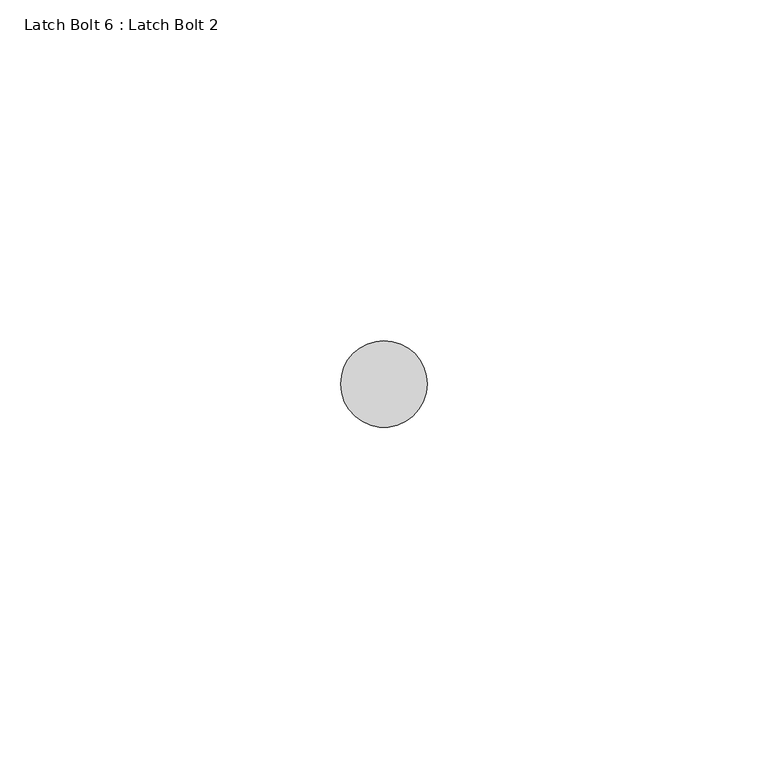
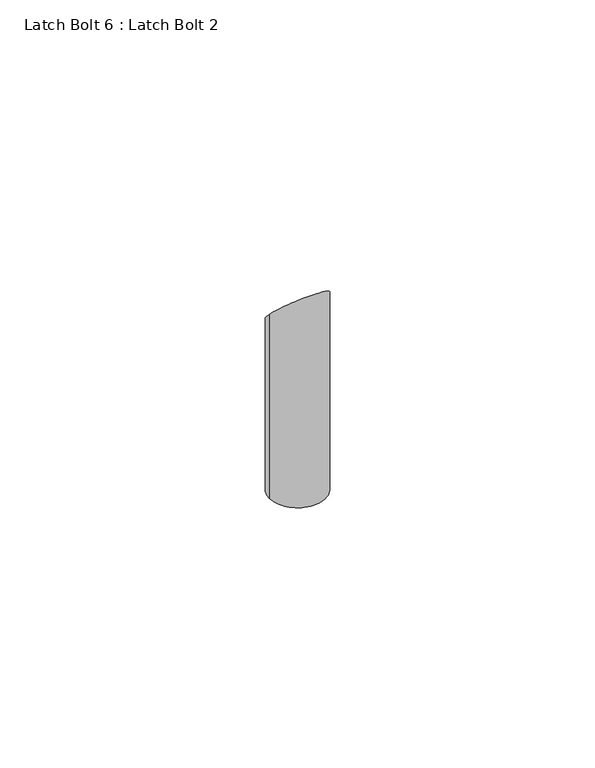
"""IFC4 building model written with IfcOpenShell, lengths in millimetres: proxy geometry, Latch Bolt 6 : Latch Bolt 2."""

from ifc_helpers import new_model, si_unit, frame, origin, place, context, project, spatial, circle_curve, ellipse_curve, source, transform, mapped, element, save
from ifc_brep_helpers import plane_surface, cylinder_surface, advanced_brep


def latch_bolt_6_latch_bolt_2_5f3dc6ce(model_context):
    return source(origin(), model_context, "Body", "AdvancedBrep", [
        advanced_brep(
        [(587306.3384816, -535293.641467, 1022.35), (587319.0384816, -535293.641467, 1022.35), (587319.0384816, -535293.641467, 1066.7505507), (587306.3384816, -535293.641467, 1066.7505507), (587312.6884816, -535287.291467, 1060.4005507)],
        [
            (0, 1, circle_curve(frame((587312.6884816, -535293.641467, 1022.35), z_axis=(0.0, 0.0, -1.0), x_axis=(1.0, 0.0, 0.0)), 6.35)),
            (1, 0, circle_curve(frame((587312.6884816, -535293.641467, 1022.35), z_axis=(0.0, 0.0, -1.0), x_axis=(1.0, 0.0, 0.0)), 6.35)),
            (1, 2),
            (2, 3, ellipse_curve(frame((587312.6884816, -535293.641467, 1066.7505507), z_axis=(0.0, -0.7071067811861375, -0.7071067811869577), x_axis=(0.0, -0.7071067811869577, 0.7071067811861372)), 8.9802561, 6.35)),
            (3, 0),
            (3, 4, ellipse_curve(frame((587312.6884816, -535293.641467, 1066.7505507), z_axis=(0.0, -0.7071067811861375, -0.7071067811869577), x_axis=(0.0, -0.7071067811869577, 0.7071067811861372)), 8.9802561, 6.35)),
            (4, 2, ellipse_curve(frame((587312.6884816, -535293.641467, 1066.7505507), z_axis=(0.0, -0.7071067811861375, -0.7071067811869577), x_axis=(0.0, -0.7071067811869577, 0.7071067811861372)), 8.9802561, 6.35)),
        ],
        [
            plane_surface(frame((587319.0384816, -535293.641467, 1022.35), z_axis=(0.0, 0.0, -1.0), x_axis=(0.0, -1.0, 0.0))),
            cylinder_surface(frame((587312.6884816, -535293.641467, 1022.35), z_axis=(0.0, 0.0, 1.0), x_axis=(1.0, 0.0, 0.0)), 6.35),
            plane_surface(frame((587338.1185739, -535303.166467, 1076.2755507), z_axis=(0.0, 0.7071067811861375, 0.7071067811869577), x_axis=(-1.0, 0.0, 0.0))),
        ],
        [
            (0, [[1, 2]]),
            (1, [[-2, 3, 4, 5]]),
            (1, [[-1, -5, 6, 7, -3]]),
            (2, [[-4, -7, -6]]),
        ],
    ),
    ])


if __name__ == "__main__":
    model = new_model("IFC4")
    model_context = context("Model", 3, world=origin())
    ifc_project = project(units=[si_unit("LENGTHUNIT", "METRE", prefix="MILLI")], contexts=[model_context])
    site = spatial("IfcSite", under=ifc_project)
    building = spatial("IfcBuilding", under=site)
    placement = place(None, origin())
    latch_bolt_6_latch_bolt_2_shape = latch_bolt_6_latch_bolt_2_5f3dc6ce(model_context)
    element("IfcBuildingElementProxy", 1, Name="Latch Bolt 6 : Latch Bolt 2", ObjectType="Latch Bolt 6 : Latch Bolt 2", at=placement, inside=building, context=model_context, shape_type="MappedRepresentation", body=[
        mapped(latch_bolt_6_latch_bolt_2_shape, transform((0.0, 0.0, 0.0), x_axis=(1.0, 0.0, 0.0), y_axis=(0.0, 1.0, 0.0), z_axis=(0.0, 0.0, 1.0))),
    ])
    save(model, "model.ifc")

# Revit data of these elements
# Element 1 (IfcBuildingElementProxy, "Latch Bolt 6 : Latch Bolt 2")
#   Materials on its faces: "GALV. GATE LATCH"
# Materials
#   "GALV. GATE LATCH": class "Metal", colour RGB 189 187 185, transparency 0, Description = "Carbon steel", Cost = 0
